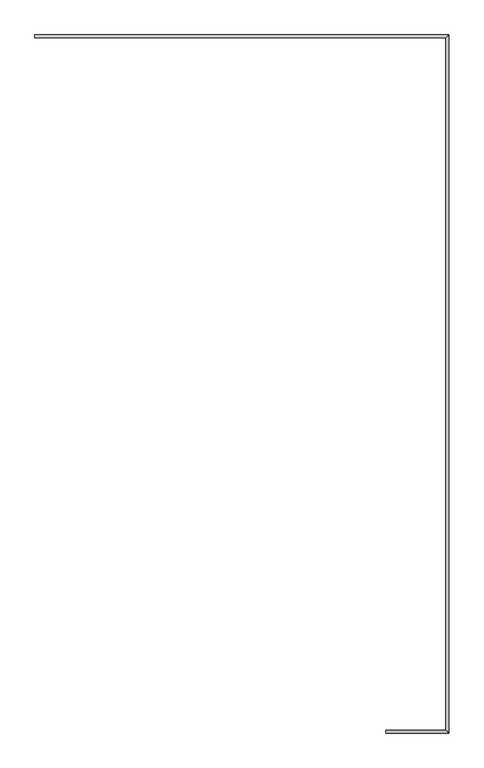
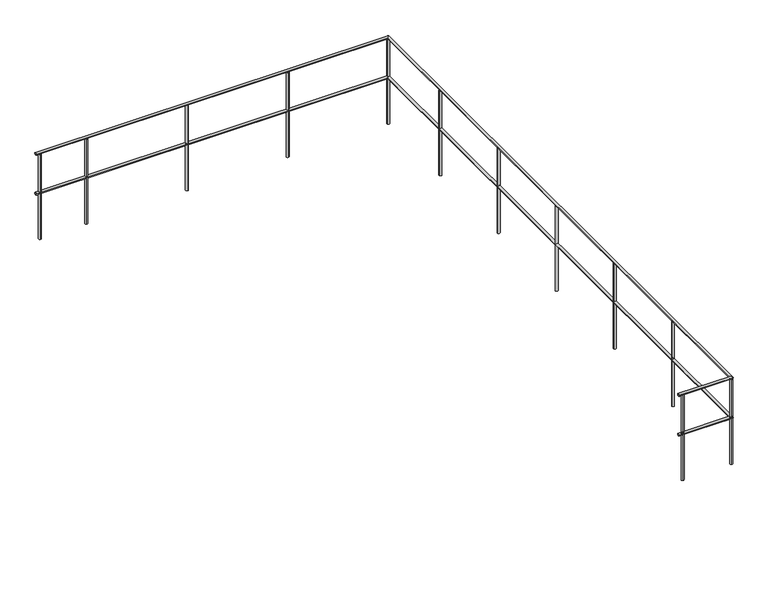
"""IFC4 building model written with IfcOpenShell, lengths in millimetres: railing geometry."""

from ifc_helpers import new_model, si_unit, point, frame, frame_2d, origin, place, context, project, spatial, circle_curve, ellipse_curve, trimmed, segment, composite_curve, outline, extrude, source, transform, mapped, element, save
from ifc_brep_helpers import plane_surface, cylinder_surface, advanced_brep


def railing_40a178cd(model_context):
    return source(origin(), model_context, "Body", "SolidModel", [
        advanced_brep(
        [(64291.0, 60942.0208589, 885.0), (64291.0, 60912.0208589, 885.0), (64904.3815191, 60942.0208589, 885.0), (64934.3815191, 60912.0208589, 885.0), (64904.3815191, 67987.0208589, 885.0), (64934.3815191, 68017.0208589, 885.0), (60716.32048, 67987.0208589, 885.0), (60716.32048, 68017.0208589, 885.0)],
        [
            (0, 1, circle_curve(frame((64291.0, 60927.0208589, 885.0), z_axis=(-1.0, 0.0, 0.0), x_axis=(0.0, -1.0, 0.0)), 15.0)),
            (1, 0, circle_curve(frame((64291.0, 60927.0208589, 885.0), z_axis=(-1.0, 0.0, 0.0), x_axis=(0.0, -1.0, 0.0)), 15.0)),
            (0, 2),
            (2, 3, ellipse_curve(frame((64919.3815191, 60927.0208589, 885.0), z_axis=(-0.7071067811865479, -0.707106781186547, 0.0), x_axis=(-0.7071067811865472, 0.7071067811865479, 0.0)), 21.2132034, 15.0)),
            (3, 1),
            (3, 2, ellipse_curve(frame((64919.3815191, 60927.0208589, 885.0), z_axis=(-0.7071067811865479, -0.707106781186547, 0.0), x_axis=(-0.7071067811865472, 0.7071067811865479, 0.0)), 21.2132034, 15.0)),
            (2, 4),
            (4, 5, ellipse_curve(frame((64919.3815191, 68002.0208589, 885.0), z_axis=(0.7071067811865456, -0.7071067811865495, 0.0), x_axis=(-0.7071067811865495, -0.7071067811865456, 0.0)), 21.2132034, 15.0)),
            (5, 3),
            (5, 4, ellipse_curve(frame((64919.3815191, 68002.0208589, 885.0), z_axis=(0.7071067811865456, -0.7071067811865495, 0.0), x_axis=(-0.7071067811865495, -0.7071067811865456, 0.0)), 21.2132034, 15.0)),
            (6, 7, circle_curve(frame((60716.32048, 68002.0208589, 885.0), z_axis=(-1.0, 0.0, 0.0), x_axis=(0.0, 1.0, 0.0)), 15.0)),
            (7, 6, circle_curve(frame((60716.32048, 68002.0208589, 885.0), z_axis=(-1.0, 0.0, 0.0), x_axis=(0.0, 1.0, 0.0)), 15.0)),
            (4, 6),
            (7, 5),
        ],
        [
            plane_surface(frame((64291.0, 60927.0208589, 900.0), z_axis=(-1.0, 0.0, 0.0), x_axis=(0.0, 1.0, 0.0))),
            cylinder_surface(frame((64291.0, 60927.0208589, 885.0), z_axis=(-1.0, 0.0, 0.0), x_axis=(0.0, -1.0, 0.0)), 15.0),
            cylinder_surface(frame((64919.3815191, 60927.0208589, 885.0), z_axis=(0.0, -1.0, 0.0), x_axis=(1.0, 0.0, 0.0)), 15.0),
            plane_surface(frame((60716.32048, 68002.0208589, 900.0), z_axis=(-1.0, 0.0, 0.0), x_axis=(0.0, -1.0, 0.0))),
            cylinder_surface(frame((64919.3815191, 68002.0208589, 885.0), z_axis=(1.0, 0.0, 0.0), x_axis=(0.0, 1.0, 0.0)), 15.0),
        ],
        [
            (0, [[1, 2]]),
            (1, [[-1, 3, 4, 5]]),
            (1, [[-2, -5, 6, -3]]),
            (2, [[-4, 7, 8, 9]]),
            (2, [[-6, -9, 10, -7]]),
            (3, [[11, 12]]),
            (4, [[-8, 13, -12, 14]]),
            (4, [[-10, -14, -11, -13]]),
        ],
    ),
        advanced_brep(
        [(64291.0, 60942.0208589, 1385.0), (64291.0, 60912.0208589, 1385.0), (64904.3815191, 60942.0208589, 1385.0), (64934.3815191, 60912.0208589, 1385.0), (64904.3815191, 67987.0208589, 1385.0), (64934.3815191, 68017.0208589, 1385.0), (60716.32048, 67987.0208589, 1385.0), (60716.32048, 68017.0208589, 1385.0)],
        [
            (0, 1, circle_curve(frame((64291.0, 60927.0208589, 1385.0), z_axis=(-1.0, 0.0, 0.0), x_axis=(0.0, -1.0, 0.0)), 15.0)),
            (1, 0, circle_curve(frame((64291.0, 60927.0208589, 1385.0), z_axis=(-1.0, 0.0, 0.0), x_axis=(0.0, -1.0, 0.0)), 15.0)),
            (0, 2),
            (2, 3, ellipse_curve(frame((64919.3815191, 60927.0208589, 1385.0), z_axis=(-0.7071067811865479, -0.707106781186547, 0.0), x_axis=(-0.7071067811865472, 0.7071067811865479, 0.0)), 21.2132034, 15.0)),
            (3, 1),
            (3, 2, ellipse_curve(frame((64919.3815191, 60927.0208589, 1385.0), z_axis=(-0.7071067811865479, -0.707106781186547, 0.0), x_axis=(-0.7071067811865472, 0.7071067811865479, 0.0)), 21.2132034, 15.0)),
            (2, 4),
            (4, 5, ellipse_curve(frame((64919.3815191, 68002.0208589, 1385.0), z_axis=(0.7071067811865456, -0.7071067811865495, 0.0), x_axis=(-0.7071067811865495, -0.7071067811865456, 0.0)), 21.2132034, 15.0)),
            (5, 3),
            (5, 4, ellipse_curve(frame((64919.3815191, 68002.0208589, 1385.0), z_axis=(0.7071067811865456, -0.7071067811865495, 0.0), x_axis=(-0.7071067811865495, -0.7071067811865456, 0.0)), 21.2132034, 15.0)),
            (6, 7, circle_curve(frame((60716.32048, 68002.0208589, 1385.0), z_axis=(-1.0, 0.0, 0.0), x_axis=(0.0, 1.0, 0.0)), 15.0)),
            (7, 6, circle_curve(frame((60716.32048, 68002.0208589, 1385.0), z_axis=(-1.0, 0.0, 0.0), x_axis=(0.0, 1.0, 0.0)), 15.0)),
            (4, 6),
            (7, 5),
        ],
        [
            plane_surface(frame((64291.0, 60927.0208589, 1400.0), z_axis=(-1.0, 0.0, 0.0), x_axis=(0.0, 1.0, 0.0))),
            cylinder_surface(frame((64291.0, 60927.0208589, 1385.0), z_axis=(-1.0, 0.0, 0.0), x_axis=(0.0, -1.0, 0.0)), 15.0),
            cylinder_surface(frame((64919.3815191, 60927.0208589, 1385.0), z_axis=(0.0, -1.0, 0.0), x_axis=(1.0, 0.0, 0.0)), 15.0),
            plane_surface(frame((60716.32048, 68002.0208589, 1400.0), z_axis=(-1.0, 0.0, 0.0), x_axis=(0.0, -1.0, 0.0))),
            cylinder_surface(frame((64919.3815191, 68002.0208589, 1385.0), z_axis=(1.0, 0.0, 0.0), x_axis=(0.0, 1.0, 0.0)), 15.0),
        ],
        [
            (0, [[1, 2]]),
            (1, [[-1, 3, 4, 5]]),
            (1, [[-2, -5, 6, -3]]),
            (2, [[-4, 7, 8, 9]]),
            (2, [[-6, -9, 10, -7]]),
            (3, [[11, 12]]),
            (4, [[-8, 13, -12, 14]]),
            (4, [[-10, -14, -11, -13]]),
        ],
    ),
        extrude(outline(composite_curve([segment(trimmed(circle_curve(frame_2d((61319.3815191, 68002.0208589)), 15.0), [point((61319.3815191, 67987.0208589))], [point((61319.3815191, 68017.0208589))], False, "CARTESIAN"), True, "CONTINUOUS"), segment(trimmed(circle_curve(frame_2d((61319.3815191, 68002.0208589)), 15.0), [point((61319.3815191, 68017.0208589))], [point((61319.3815191, 67987.0208589))], False, "CARTESIAN"), True, "CONTINUOUS")], self_intersect=False)), frame((0.0, 0.0, 300.0), z_axis=(0.0, 0.0, 1.0), x_axis=(1.0, 0.0, 0.0)), (0.0, 0.0, 1.0), 1070.0),
        extrude(outline(composite_curve([segment(trimmed(circle_curve(frame_2d((62519.3815191, 68002.0208589)), 15.0), [point((62519.3815191, 67987.0208589))], [point((62519.3815191, 68017.0208589))], False, "CARTESIAN"), True, "CONTINUOUS"), segment(trimmed(circle_curve(frame_2d((62519.3815191, 68002.0208589)), 15.0), [point((62519.3815191, 68017.0208589))], [point((62519.3815191, 67987.0208589))], False, "CARTESIAN"), True, "CONTINUOUS")], self_intersect=False)), frame((0.0, 0.0, 300.0), z_axis=(0.0, 0.0, 1.0), x_axis=(1.0, 0.0, 0.0)), (0.0, 0.0, 1.0), 1070.0),
        extrude(outline(composite_curve([segment(trimmed(circle_curve(frame_2d((63719.3815191, 68002.0208589)), 15.0), [point((63719.3815191, 67987.0208589))], [point((63719.3815191, 68017.0208589))], False, "CARTESIAN"), True, "CONTINUOUS"), segment(trimmed(circle_curve(frame_2d((63719.3815191, 68002.0208589)), 15.0), [point((63719.3815191, 68017.0208589))], [point((63719.3815191, 67987.0208589))], False, "CARTESIAN"), True, "CONTINUOUS")], self_intersect=False)), frame((0.0, 0.0, 300.0), z_axis=(0.0, 0.0, 1.0), x_axis=(1.0, 0.0, 0.0)), (0.0, 0.0, 1.0), 1070.0),
        extrude(outline(composite_curve([segment(trimmed(circle_curve(frame_2d((64919.3815191, 66927.0208589)), 15.0), [point((64904.3815191, 66927.0208589))], [point((64934.3815191, 66927.0208589))], False, "CARTESIAN"), True, "CONTINUOUS"), segment(trimmed(circle_curve(frame_2d((64919.3815191, 66927.0208589)), 15.0), [point((64934.3815191, 66927.0208589))], [point((64904.3815191, 66927.0208589))], False, "CARTESIAN"), True, "CONTINUOUS")], self_intersect=False)), frame((0.0, 0.0, 300.0), z_axis=(0.0, 0.0, 1.0), x_axis=(1.0, 0.0, 0.0)), (0.0, 0.0, 1.0), 1070.0),
        extrude(outline(composite_curve([segment(trimmed(circle_curve(frame_2d((64919.3815191, 65727.0208589)), 15.0), [point((64904.3815191, 65727.0208589))], [point((64934.3815191, 65727.0208589))], False, "CARTESIAN"), True, "CONTINUOUS"), segment(trimmed(circle_curve(frame_2d((64919.3815191, 65727.0208589)), 15.0), [point((64934.3815191, 65727.0208589))], [point((64904.3815191, 65727.0208589))], False, "CARTESIAN"), True, "CONTINUOUS")], self_intersect=False)), frame((0.0, 0.0, 300.0), z_axis=(0.0, 0.0, 1.0), x_axis=(1.0, 0.0, 0.0)), (0.0, 0.0, 1.0), 1070.0),
        extrude(outline(composite_curve([segment(trimmed(circle_curve(frame_2d((64919.3815191, 64527.0208589)), 15.0), [point((64904.3815191, 64527.0208589))], [point((64934.3815191, 64527.0208589))], False, "CARTESIAN"), True, "CONTINUOUS"), segment(trimmed(circle_curve(frame_2d((64919.3815191, 64527.0208589)), 15.0), [point((64934.3815191, 64527.0208589))], [point((64904.3815191, 64527.0208589))], False, "CARTESIAN"), True, "CONTINUOUS")], self_intersect=False)), frame((0.0, 0.0, 300.0), z_axis=(0.0, 0.0, 1.0), x_axis=(1.0, 0.0, 0.0)), (0.0, 0.0, 1.0), 1070.0),
        extrude(outline(composite_curve([segment(trimmed(circle_curve(frame_2d((64919.3815191, 63327.0208589)), 15.0), [point((64904.3815191, 63327.0208589))], [point((64934.3815191, 63327.0208589))], False, "CARTESIAN"), True, "CONTINUOUS"), segment(trimmed(circle_curve(frame_2d((64919.3815191, 63327.0208589)), 15.0), [point((64934.3815191, 63327.0208589))], [point((64904.3815191, 63327.0208589))], False, "CARTESIAN"), True, "CONTINUOUS")], self_intersect=False)), frame((0.0, 0.0, 300.0), z_axis=(0.0, 0.0, 1.0), x_axis=(1.0, 0.0, 0.0)), (0.0, 0.0, 1.0), 1070.0),
        extrude(outline(composite_curve([segment(trimmed(circle_curve(frame_2d((64919.3815191, 62127.0208589)), 15.0), [point((64904.3815191, 62127.0208589))], [point((64934.3815191, 62127.0208589))], False, "CARTESIAN"), True, "CONTINUOUS"), segment(trimmed(circle_curve(frame_2d((64919.3815191, 62127.0208589)), 15.0), [point((64934.3815191, 62127.0208589))], [point((64904.3815191, 62127.0208589))], False, "CARTESIAN"), True, "CONTINUOUS")], self_intersect=False)), frame((0.0, 0.0, 300.0), z_axis=(0.0, 0.0, 1.0), x_axis=(1.0, 0.0, 0.0)), (0.0, 0.0, 1.0), 1070.0),
        extrude(outline(composite_curve([segment(trimmed(circle_curve(frame_2d((64919.3815191, 68002.0208589)), 15.0), [point((64904.3815191, 68002.0208589))], [point((64934.3815191, 68002.0208589))], False, "CARTESIAN"), True, "CONTINUOUS"), segment(trimmed(circle_curve(frame_2d((64919.3815191, 68002.0208589)), 15.0), [point((64934.3815191, 68002.0208589))], [point((64904.3815191, 68002.0208589))], False, "CARTESIAN"), True, "CONTINUOUS")], self_intersect=False)), frame((0.0, 0.0, 300.0), z_axis=(0.0, 0.0, 1.0), x_axis=(1.0, 0.0, 0.0)), (0.0, 0.0, 1.0), 1070.0),
        extrude(outline(composite_curve([segment(trimmed(circle_curve(frame_2d((64919.3815191, 60927.0208589)), 15.0), [point((64919.3815191, 60942.0208589))], [point((64919.3815191, 60912.0208589))], False, "CARTESIAN"), True, "CONTINUOUS"), segment(trimmed(circle_curve(frame_2d((64919.3815191, 60927.0208589)), 15.0), [point((64919.3815191, 60912.0208589))], [point((64919.3815191, 60942.0208589))], False, "CARTESIAN"), True, "CONTINUOUS")], self_intersect=False)), frame((0.0, 0.0, 300.0), z_axis=(0.0, 0.0, 1.0), x_axis=(1.0, 0.0, 0.0)), (0.0, 0.0, 1.0), 1070.0),
        extrude(outline(composite_curve([segment(trimmed(circle_curve(frame_2d((60766.32048, 68002.0208589)), 15.0), [point((60766.32048, 67987.0208589))], [point((60766.32048, 68017.0208589))], False, "CARTESIAN"), True, "CONTINUOUS"), segment(trimmed(circle_curve(frame_2d((60766.32048, 68002.0208589)), 15.0), [point((60766.32048, 68017.0208589))], [point((60766.32048, 67987.0208589))], False, "CARTESIAN"), True, "CONTINUOUS")], self_intersect=False)), frame((0.0, 0.0, 300.0), z_axis=(0.0, 0.0, 1.0), x_axis=(1.0, 0.0, 0.0)), (0.0, 0.0, 1.0), 1070.0),
        extrude(outline(composite_curve([segment(trimmed(circle_curve(frame_2d((64341.0, 60927.0208589)), 15.0), [point((64341.0, 60942.0208589))], [point((64341.0, 60912.0208589))], False, "CARTESIAN"), True, "CONTINUOUS"), segment(trimmed(circle_curve(frame_2d((64341.0, 60927.0208589)), 15.0), [point((64341.0, 60912.0208589))], [point((64341.0, 60942.0208589))], False, "CARTESIAN"), True, "CONTINUOUS")], self_intersect=False)), frame((0.0, 0.0, 300.0), z_axis=(0.0, 0.0, 1.0), x_axis=(1.0, 0.0, 0.0)), (0.0, 0.0, 1.0), 1070.0),
    ])


if __name__ == "__main__":
    model = new_model("IFC4")
    model_context = context("Model", 3, world=origin())
    ifc_project = project(units=[si_unit("LENGTHUNIT", "METRE", prefix="MILLI")], contexts=[model_context])
    site = spatial("IfcSite", under=ifc_project)
    building = spatial("IfcBuilding", under=site)
    placement = place(None, origin())
    railing_shape = railing_40a178cd(model_context)
    element("IfcRailing", 1, at=placement, inside=building, context=model_context, shape_type="MappedRepresentation", body=[
        mapped(railing_shape, transform((0.0, 0.0, 0.0), x_axis=(1.0, 0.0, 0.0), y_axis=(0.0, 1.0, 0.0), z_axis=(0.0, 0.0, 1.0))),
    ])
    save(model, "model.ifc")
